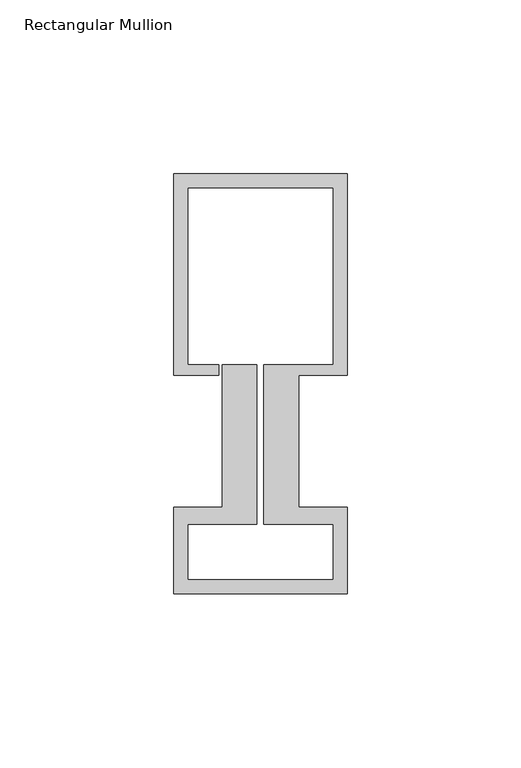
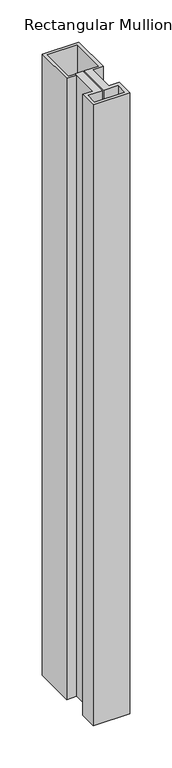
"""IFC4 building model written with IfcOpenShell, lengths in millimetres: member geometry, Rectangular Mullion : Schueco_FWS-50-SI_Tran_CovCap-20mm_Tran-55mm."""

from ifc_helpers import new_model, si_unit, frame, origin, place, context, project, spatial, polyline, outline, extrude, source, transform, mapped, element, save


def rectangular_mullion_d26f1b66(model_context):
    return source(origin(), model_context, "Body", "SweptSolid", [
        extrude(outline(polyline([(0.0, 96.0), (0.0, 38.0), (-14.0, 38.0), (-14.0, -0.1), (0.0, -0.1), (0.0, -25.0), (-50.0, -25.0), (-50.0, -0.1), (-36.0, -0.1), (-36.0, 41.0), (-26.0, 41.0), (-26.0, -5.0), (-46.0, -5.0), (-46.0, -21.0), (-4.0, -21.0), (-4.0, -5.0), (-24.0, -5.0), (-24.0, 41.0), (-4.0, 41.0), (-4.0, 92.0), (-46.0, 92.0), (-46.0, 41.0), (-37.0, 41.0), (-37.0, 38.0), (-50.0, 38.0), (-50.0, 96.0), (0.0, 96.0)])), frame((0.0, 0.0, -900.0), z_axis=(0.0, 0.0, 1.0), x_axis=(1.0, 0.0, 0.0)), (0.0, 0.0, 1.0), 900.0),
    ])


if __name__ == "__main__":
    model = new_model("IFC4")
    model_context = context("Model", 3, world=origin())
    ifc_project = project(units=[si_unit("LENGTHUNIT", "METRE", prefix="MILLI")], contexts=[model_context])
    site = spatial("IfcSite", under=ifc_project)
    building = spatial("IfcBuilding", under=site)
    placement = place(None, origin())
    rectangular_mullion_shape = rectangular_mullion_d26f1b66(model_context)
    element("IfcMember", 1, ObjectType="Rectangular Mullion : Schueco_FWS-50-SI_Tran_CovCap-20mm_Tran-55mm", at=placement, inside=building, context=model_context, shape_type="MappedRepresentation", body=[
        mapped(rectangular_mullion_shape, transform((0.0, 0.0, 0.0), x_axis=(1.0, 0.0, 0.0), y_axis=(0.0, 1.0, 0.0), z_axis=(0.0, 0.0, 1.0))),
    ])
    save(model, "model.ifc")

# Revit data of these elements
# Type "Rectangular Mullion : Schueco_FWS-50-SI_Tran_CovCap-20mm_Tran-55mm"
#   Model = "FWS 50.SI"
#   Manufacturer = "Schueco International KG"
#   Type Comments = "Transom"
#   Schueco thermal insulation standard = "Suitable for passive houses"
#   Burglar resistance = "RC 3"
#   Thermal insulation = "to 0.70 W/(m²K)"
#   built-in parameter 1007322 = 0.396982 (stored number, unit not read)
#   built-in parameter 1007321 = 0.0360892 (stored number, unit not read)
#   built-in parameter 1007320 = 0.0360892 (stored number, unit not read)
# Element 1 (IfcMember, "Rectangular Mullion : Schueco_FWS-50-SI_Tran_CovCap-20mm_Tran-55mm")
#   Materials on its faces: "Alu"
# Materials
#   "Alu": class "Glas", colour RGB 140 140 140, transparency 0
